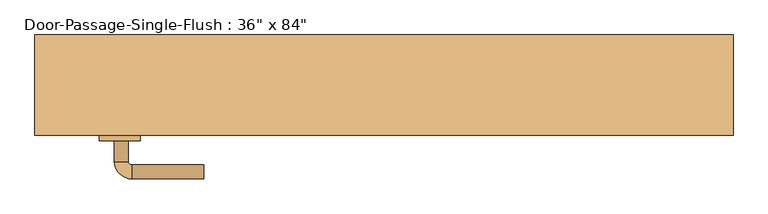
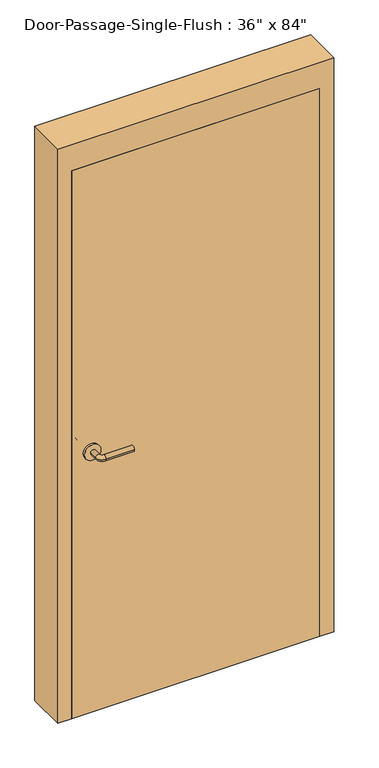
"""IFC4 building model written with IfcOpenShell, lengths in millimetres: door geometry."""

from ifc_helpers import new_model, si_unit, point, frame, frame_2d, origin, origin_with_axes, place, context, project, spatial, polyline, circle_curve, ellipse_curve, trimmed, segment, composite_curve, outline, extrude, faceted_brep, source, transform, mapped, element, save
from ifc_brep_helpers import plane_surface, cylinder_surface, revolved_surface, advanced_brep


def door_5b314290(model_context):
    return source(origin(), model_context, "Body", "SolidModel", [
        advanced_brep(
        [(-392.190625, 1.65, 1016.0), (-372.190625, 1.65, 1016.0), (-392.190625, 31.65, 1016.0), (-372.190625, 31.65, 1016.0), (-367.190625, 36.65, 1016.0), (-367.190625, 56.65, 1016.0), (-262.190625, 56.65, 1016.0), (-262.190625, 36.65, 1016.0)],
        [
            (0, 1, circle_curve(frame((-382.190625, 1.65, 1016.0), z_axis=(0.0, -1.0, 0.0), x_axis=(1.0, 0.0, 0.0)), 10.0)),
            (1, 0, circle_curve(frame((-382.190625, 1.65, 1016.0), z_axis=(0.0, -1.0, 0.0), x_axis=(1.0, 0.0, 0.0)), 10.0)),
            (0, 2),
            (2, 3, circle_curve(frame((-382.190625, 31.65, 1016.0), z_axis=(0.0, -1.0, 0.0), x_axis=(1.0, 0.0, 0.0)), 10.0)),
            (3, 1),
            (3, 2, circle_curve(frame((-382.190625, 31.65, 1016.0), z_axis=(0.0, -1.0, 0.0), x_axis=(1.0, 0.0, 0.0)), 10.0)),
            (4, 3, circle_curve(frame((-367.190625, 31.65, 1016.0), z_axis=(0.0, 0.0, 1.0), x_axis=(-1.0, 0.0, 0.0)), 5.0)),
            (2, 5, circle_curve(frame((-367.190625, 31.65, 1016.0), z_axis=(0.0, 0.0, -1.0), x_axis=(-1.0, 0.0, 0.0)), 25.0)),
            (5, 4, circle_curve(frame((-367.190625, 46.65, 1016.0), z_axis=(-1.0, 0.0, 0.0), x_axis=(0.0, -1.0, 0.0)), 10.0)),
            (4, 5, circle_curve(frame((-367.190625, 46.65, 1016.0), z_axis=(-1.0, 0.0, 0.0), x_axis=(0.0, -1.0, 0.0)), 10.0)),
            (6, 7, circle_curve(frame((-262.190625, 46.65, 1016.0), z_axis=(1.0, 0.0, 0.0), x_axis=(0.0, -1.0, 0.0)), 10.0)),
            (7, 6, circle_curve(frame((-262.190625, 46.65, 1016.0), z_axis=(1.0, 0.0, 0.0), x_axis=(0.0, -1.0, 0.0)), 10.0)),
            (5, 6),
            (7, 4),
        ],
        [
            plane_surface(frame((-382.190625, 1.65, 1016.0), z_axis=(0.0, -1.0, 0.0), x_axis=(0.0, 0.0, 1.0))),
            cylinder_surface(frame((-382.190625, 1.65, 1016.0), z_axis=(0.0, -1.0, 0.0), x_axis=(1.0, 0.0, 0.0)), 10.0),
            revolved_surface(trimmed(ellipse_curve(frame((-382.190625, 31.65, 1016.0), z_axis=(0.0, -1.0, 0.0), x_axis=(1.0, 0.0, 0.0)), 10.0, 10.0), [point((-392.190625, 31.65, 1016.0))], [point((-372.190625, 31.65, 1016.0))], True, "CARTESIAN"), (-367.190625, 31.65, 1016.0), (0.0, 0.0, -1.0)),
            revolved_surface(trimmed(ellipse_curve(frame((-382.190625, 31.65, 1016.0), z_axis=(0.0, -1.0, 0.0), x_axis=(1.0, 0.0, 0.0)), 10.0, 10.0), [point((-372.190625, 31.65, 1016.0))], [point((-392.190625, 31.65, 1016.0))], True, "CARTESIAN"), (-367.190625, 31.65, 1016.0), (0.0, 0.0, -1.0)),
            plane_surface(frame((-262.190625, 46.65, 1016.0), z_axis=(1.0, 0.0, 0.0), x_axis=(0.0, 0.0, 1.0))),
            cylinder_surface(frame((-367.190625, 46.65, 1016.0), z_axis=(-1.0, 0.0, 0.0), x_axis=(0.0, -1.0, 0.0)), 10.0),
        ],
        [
            (0, [[1, 2]]),
            (1, [[-1, 3, 4, 5]]),
            (1, [[-2, -5, 6, -3]]),
            (2, [[7, -4, 8, 9]]),
            (3, [[-8, -6, -7, 10]]),
            (4, [[11, 12]]),
            (5, [[-9, 13, -12, 14]]),
            (5, [[-10, -14, -11, -13]]),
        ],
    ),
        extrude(outline(composite_curve([segment(trimmed(circle_curve(frame_2d((1016.0, -384.690625)), 30.0), [point((1016.0, -414.690625))], [point((1016.0, -354.690625))], False, "CARTESIAN"), True, "CONTINUOUS"), segment(trimmed(circle_curve(frame_2d((1016.0, -384.690625)), 30.0), [point((1016.0, -354.690625))], [point((1016.0, -414.690625))], False, "CARTESIAN"), True, "CONTINUOUS")], self_intersect=False)), frame((0.0, -6.35, 0.0), z_axis=(0.0, 1.0, 0.0), x_axis=(0.0, 0.0, 1.0)), (0.0, 0.0, 1.0), 8.0),
        advanced_brep(
        [(-392.190625, -58.8, 1016.0), (-372.190625, -58.8, 1016.0), (-372.190625, -88.8, 1016.0), (-392.190625, -88.8, 1016.0), (-367.190625, -93.8, 1016.0), (-367.190625, -113.8, 1016.0), (-262.190625, -113.8, 1016.0), (-262.190625, -93.8, 1016.0)],
        [
            (0, 1, circle_curve(frame((-382.190625, -58.8, 1016.0), z_axis=(0.0, 1.0, 0.0), x_axis=(1.0, 0.0, 0.0)), 10.0)),
            (1, 0, circle_curve(frame((-382.190625, -58.8, 1016.0), z_axis=(0.0, 1.0, 0.0), x_axis=(1.0, 0.0, 0.0)), 10.0)),
            (1, 2),
            (2, 3, circle_curve(frame((-382.190625, -88.8, 1016.0), z_axis=(0.0, 1.0, 0.0), x_axis=(1.0, 0.0, 0.0)), 10.0)),
            (3, 0),
            (3, 2, circle_curve(frame((-382.190625, -88.8, 1016.0), z_axis=(0.0, 1.0, 0.0), x_axis=(1.0, 0.0, 0.0)), 10.0)),
            (4, 5, circle_curve(frame((-367.190625, -103.8, 1016.0), z_axis=(-1.0, 0.0, 0.0), x_axis=(0.0, 1.0, 0.0)), 10.0)),
            (5, 3, circle_curve(frame((-367.190625, -88.8, 1016.0), z_axis=(0.0, 0.0, -1.0), x_axis=(-1.0, 0.0, 0.0)), 25.0)),
            (2, 4, circle_curve(frame((-367.190625, -88.8, 1016.0), z_axis=(0.0, 0.0, 1.0), x_axis=(-1.0, 0.0, 0.0)), 5.0)),
            (5, 4, circle_curve(frame((-367.190625, -103.8, 1016.0), z_axis=(-1.0, 0.0, 0.0), x_axis=(0.0, 1.0, 0.0)), 10.0)),
            (6, 7, circle_curve(frame((-262.190625, -103.8, 1016.0), z_axis=(1.0, 0.0, 0.0), x_axis=(0.0, 1.0, 0.0)), 10.0)),
            (7, 6, circle_curve(frame((-262.190625, -103.8, 1016.0), z_axis=(1.0, 0.0, 0.0), x_axis=(0.0, 1.0, 0.0)), 10.0)),
            (4, 7),
            (6, 5),
        ],
        [
            plane_surface(frame((-382.190625, -58.8, 1016.0), z_axis=(0.0, 1.0, 0.0), x_axis=(0.0, 0.0, 1.0))),
            cylinder_surface(frame((-382.190625, -58.8, 1016.0), z_axis=(0.0, 1.0, 0.0), x_axis=(1.0, 0.0, 0.0)), 10.0),
            revolved_surface(trimmed(ellipse_curve(frame((-382.190625, -88.8, 1016.0), z_axis=(0.0, -1.0, 0.0), x_axis=(1.0, 0.0, 0.0)), 10.0, 10.0), [point((-392.190625, -88.8, 1016.0))], [point((-372.190625, -88.8, 1016.0))], True, "CARTESIAN"), (-367.190625, -88.8, 1016.0), (0.0, 0.0, -1.0)),
            revolved_surface(trimmed(ellipse_curve(frame((-382.190625, -88.8, 1016.0), z_axis=(0.0, -1.0, 0.0), x_axis=(1.0, 0.0, 0.0)), 10.0, 10.0), [point((-372.190625, -88.8, 1016.0))], [point((-392.190625, -88.8, 1016.0))], True, "CARTESIAN"), (-367.190625, -88.8, 1016.0), (0.0, 0.0, -1.0)),
            plane_surface(frame((-262.190625, -103.8, 1016.0), z_axis=(1.0, 0.0, 0.0), x_axis=(0.0, 0.0, 1.0))),
            cylinder_surface(frame((-367.190625, -103.8, 1016.0), z_axis=(-1.0, 0.0, 0.0), x_axis=(0.0, 1.0, 0.0)), 10.0),
        ],
        [
            (0, [[1, 2]]),
            (1, [[3, 4, 5, -2]]),
            (1, [[-5, 6, -3, -1]]),
            (2, [[7, 8, -4, 9]]),
            (3, [[10, -9, -6, -8]]),
            (4, [[11, 12]]),
            (5, [[13, -11, 14, -7]]),
            (5, [[-14, -12, -13, -10]]),
        ],
    ),
        extrude(outline(composite_curve([segment(trimmed(circle_curve(frame_2d((1016.0, -384.690625)), 30.0), [point((1016.0, -414.690625))], [point((1016.0, -354.690625))], False, "CARTESIAN"), True, "CONTINUOUS"), segment(trimmed(circle_curve(frame_2d((1016.0, -384.690625)), 30.0), [point((1016.0, -354.690625))], [point((1016.0, -414.690625))], False, "CARTESIAN"), True, "CONTINUOUS")], self_intersect=False)), frame((0.0, -58.8, 0.0), z_axis=(0.0, 1.0, 0.0), x_axis=(0.0, 0.0, 1.0)), (0.0, 0.0, 1.0), 8.0),
        faceted_brep([(457.2, -1.5875, 0.0), (441.325, -1.5875, 0.0), (441.325, 46.0375, 0.0), (457.2, 46.0375, 0.0), (457.2, 95.25, 0.0), (508.0, 95.25, 0.0), (508.0, -50.8, 0.0), (457.2, -50.8, 0.0), (457.2, -50.8, 2133.6), (457.2, -1.5875, 2133.6), (508.0, -50.8, 2235.2), (-508.0, -50.8, 2235.2), (-508.0, -50.8, 0.0), (-457.2, -50.8, 0.0), (-457.2, -50.8, 2133.6), (508.0, 95.25, 2235.2), (457.2, 95.25, 2133.6), (-457.2, 95.25, 2133.6), (-457.2, 95.25, 0.0), (-508.0, 95.25, 0.0), (-508.0, 95.25, 2235.2), (457.2, 46.0375, 2133.6), (441.325, 46.0375, 2117.725), (-441.325, 46.0375, 2117.725), (-441.325, 46.0375, 0.0), (-457.2, 46.0375, 0.0), (-457.2, 46.0375, 2133.6), (441.325, -1.5875, 2117.725), (-457.2, -1.5875, 2133.6), (-457.2, -1.5875, 0.0), (-441.325, -1.5875, 0.0), (-441.325, -1.5875, 2117.725)], [[[0, 1, 2, 3, 4, 5, 6, 7]], [[7, 8, 9, 0]], [[6, 10, 11, 12, 13, 14, 8, 7]], [[5, 15, 10, 6]], [[4, 16, 17, 18, 19, 20, 15, 5]], [[3, 21, 16, 4]], [[2, 22, 23, 24, 25, 26, 21, 3]], [[1, 27, 22, 2]], [[0, 9, 28, 29, 30, 31, 27, 1]], [[8, 14, 28, 9]], [[16, 21, 26, 17]], [[22, 27, 31, 23]], [[12, 19, 18, 25, 24, 30, 29, 13]], [[13, 29, 28, 14]], [[11, 20, 19, 12]], [[17, 26, 25, 18]], [[23, 31, 30, 24]], [[15, 20, 11, 10]]]),
        extrude(outline(polyline([(457.2, -6.35), (457.2, -50.8), (-457.2, -50.8), (-457.2, -6.35), (457.2, -6.35)])), origin_with_axes(), (0.0, 0.0, 1.0), 2133.6),
    ])


if __name__ == "__main__":
    model = new_model("IFC4")
    model_context = context("Model", 3, world=origin())
    ifc_project = project(units=[si_unit("LENGTHUNIT", "METRE", prefix="MILLI")], contexts=[model_context])
    site = spatial("IfcSite", under=ifc_project)
    building = spatial("IfcBuilding", under=site)
    placement = place(None, origin())
    door_shape = door_5b314290(model_context)
    element("IfcDoor", 1, ObjectType="Door-Passage-Single-Flush : 36\" x 84\"", at=placement, inside=building, context=model_context, shape_type="MappedRepresentation", body=[
        mapped(door_shape, transform((0.0, 0.0, 0.0), x_axis=(1.0, 0.0, 0.0), y_axis=(0.0, 1.0, 0.0), z_axis=(0.0, 0.0, 1.0))),
    ])
    save(model, "model.ifc")

# Revit data of these elements
# Type "Door-Passage-Single-Flush : 36\" x 84\""
#   Type Mark = "35"
#   Assembly Code = "B2030200"
#   Analytic Construction = "Wooden"
#   Thickness = 0' - 1 3/4"
#   Thermal Resistance (R) = 2.5876 (h·ft²·°F)/BTU
#   Swing Angle [instance default] = 90.00°
#   Strike Height = 3' - 4"
#   Rough Width [instance default] = 3' - 4"
#   Rough Height [instance default] = 7' - 4"
#   MF Opening Height [instance default] = 0' - 4"
#   MF Opening Width [instance default] = 0' - 4"
#   Inset Calculate [instance default] = 0' - 4"
#   Masonry Inset [instance default] = 0' - 1"
#   Height = 7' - 0"
#   Width = 3' - 0"
#   Heat Transfer Coefficient (U) = 0.3865 BTU/(h·ft²·°F)
#   Masonry Frame Depth = 0' - 5 3/4"
#   Masonry Frame [instance default] = yes
#   Function = 1
#   Dry Wall Frame [instance default] = no
#   Panel Material = Wood - Birch
#   Frame Material = Metal - Paint Finish - Grey
#   Door Handle Material = Aluminum
#   Visual Light Transmittance = 0
#   Solar Heat Gain Coefficient = 0
#   Wall Closure = (empty or 0)
# Element 1 (IfcDoor, "Door-Passage-Single-Flush : 36\" x 84\"")
#   Materials on its faces: "Aluminum", "Metal - Paint Finish - Grey", "Wood - Birch"
# Materials
#   "Wood - Birch": class "Wood", colour RGB 166 116 52, transparency 0, Cost = 0
#   "Metal - Paint Finish - Grey": class "Paint", colour RGB 104 104 104, transparency 0, Cost = 0
#   "Aluminum": class "Metal", colour RGB 247 247 247, transparency 0, Description = "Aluminum 6061", Cost = 0
